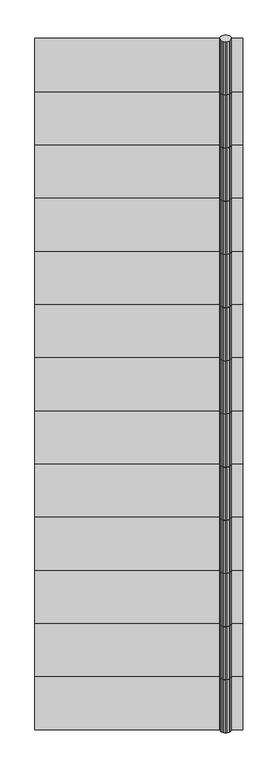
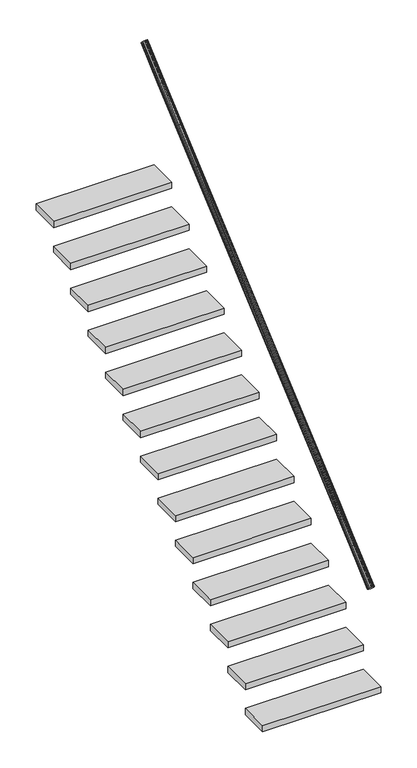
"""IFC4 building model written with IfcOpenShell, lengths in millimetres: stair geometry, 0_3d_modell."""

from ifc_helpers import new_model, si_unit, frame, origin, origin_with_axes, place, context, project, spatial, polyline, outline, extrude, source, transform, mapped, element, save


def stair_8bb973e3(model_context):
    return source(origin(), model_context, "Body", "SweptSolid", [
        extrude(outline(polyline([(1.2235871, -7.0656631), (0.0, 0.0), (1.2235871, 7.065663), (4.7745751, 13.4396897), (10.3053687, 18.498146), (17.2745751, 21.7458748), (25.0, 22.8649659), (32.7254249, 21.7458748), (39.6946313, 18.498146), (45.2254249, 13.4396897), (48.7764129, 7.065663), (50.0, 0.0), (48.7764129, -7.0656631), (45.2254249, -13.4396898), (39.6946313, -18.498146), (32.7254249, -21.7458748), (25.0, -22.8649659), (17.2745751, -21.7458748), (10.3053687, -18.498146), (4.7745751, -13.4396898), (1.2235871, -7.0656631)])), frame((850.0, 2774.9421971, 3252.4163795), z_axis=(0.0, 0.7569287102857436, 0.6534974579485071), x_axis=(-1.0, 0.0, 0.0)), (0.0, 0.0, 1.0), 303.8595272),
        extrude(outline(polyline([(0.0, 1164.9421971), (0.0, 1394.9421971), (900.0, 1394.9421971), (900.0, 1164.9421971), (0.0, 1164.9421971)])), frame((0.0, 0.0, 992.8571429), z_axis=(0.0, 0.0, 1.0), x_axis=(1.0, 0.0, 0.0)), (0.0, 0.0, 1.0), 50.0),
        extrude(outline(polyline([(0.0, 2544.9421971), (0.0, 2774.9421971), (900.0, 2774.9421971), (900.0, 2544.9421971), (0.0, 2544.9421971)])), frame((0.0, 0.0, 2184.2857143), z_axis=(0.0, 0.0, 1.0), x_axis=(1.0, 0.0, 0.0)), (0.0, 0.0, 1.0), 50.0),
        extrude(outline(polyline([(1.2235871, -7.0656631), (0.0, 0.0), (1.2235871, 7.065663), (4.7745751, 13.4396897), (10.3053687, 18.498146), (17.2745751, 21.7458748), (25.0, 22.8649659), (32.7254249, 21.7458748), (39.6946313, 18.498146), (45.2254249, 13.4396897), (48.7764129, 7.065663), (50.0, 0.0), (48.7764129, -7.0656631), (45.2254249, -13.4396897), (39.6946313, -18.498146), (32.7254249, -21.7458748), (25.0, -22.8649659), (17.2745751, -21.7458748), (10.3053687, -18.498146), (4.7745751, -13.4396897), (1.2235871, -7.0656631)])), frame((850.0, 1624.9421971, 2259.5592366), z_axis=(0.0, 0.7569287102856869, 0.653497457948573), x_axis=(-1.0, 0.0, 0.0)), (0.0, 0.0, 1.0), 303.8595272),
        extrude(outline(polyline([(1.2235871, -7.0656631), (0.0, 0.0), (1.2235871, 7.065663), (4.7745751, 13.4396898), (10.3053687, 18.498146), (17.2745751, 21.7458748), (25.0, 22.8649659), (32.7254249, 21.7458748), (39.6946313, 18.498146), (45.2254249, 13.4396898), (48.7764129, 7.065663), (50.0, 0.0), (48.7764129, -7.0656631), (45.2254249, -13.4396897), (39.6946313, -18.498146), (32.7254249, -21.7458748), (25.0, -22.8649659), (17.2745751, -21.7458748), (10.3053687, -18.498146), (4.7745751, -13.4396897), (1.2235871, -7.0656631)])), frame((850.0, 704.9421971, 1465.2735223), z_axis=(0.0, 0.7569287102857089, 0.6534974579485475), x_axis=(-1.0, 0.0, 0.0)), (0.0, 0.0, 1.0), 303.8595272),
        extrude(outline(polyline([(0.0, 244.9421971), (0.0, 474.9421971), (900.0, 474.9421971), (900.0, 244.9421971), (0.0, 244.9421971)])), frame((0.0, 0.0, 198.5714286), z_axis=(0.0, 0.0, 1.0), x_axis=(1.0, 0.0, 0.0)), (0.0, 0.0, 1.0), 50.0),
        extrude(outline(polyline([(0.0, 1624.9421971), (0.0, 1854.9421971), (900.0, 1854.9421971), (900.0, 1624.9421971), (0.0, 1624.9421971)])), frame((0.0, 0.0, 1390.0), z_axis=(0.0, 0.0, 1.0), x_axis=(1.0, 0.0, 0.0)), (0.0, 0.0, 1.0), 50.0),
        extrude(outline(polyline([(1.2235871, -7.0656631), (0.0, 0.0), (1.2235871, 7.065663), (4.7745751, 13.4396897), (10.3053687, 18.498146), (17.2745751, 21.7458748), (25.0, 22.8649659), (32.7254249, 21.7458748), (39.6946313, 18.498146), (45.2254249, 13.4396897), (48.7764129, 7.065663), (50.0, 0.0), (48.7764129, -7.0656631), (45.2254249, -13.4396898), (39.6946313, -18.498146), (32.7254249, -21.7458748), (25.0, -22.8649659), (17.2745751, -21.7458748), (10.3053687, -18.498146), (4.7745751, -13.4396898), (1.2235871, -7.0656631)])), frame((850.0, 934.9421971, 1663.8449509), z_axis=(0.0, 0.7569287102857098, 0.6534974579485463), x_axis=(-1.0, 0.0, 0.0)), (0.0, 0.0, 1.0), 303.8595272),
        extrude(outline(polyline([(1.2235871, -7.0656631), (0.0, 0.0), (1.2235871, 7.0656631), (4.7745751, 13.4396898), (10.3053687, 18.4981461), (17.2745751, 21.7458748), (25.0, 22.8649659), (32.7254249, 21.7458748), (39.6946313, 18.4981461), (45.2254249, 13.4396898), (48.7764129, 7.0656631), (50.0, 0.0), (48.7764129, -7.0656631), (45.2254249, -13.4396897), (39.6946313, -18.498146), (32.7254249, -21.7458748), (25.0, -22.8649659), (17.2745751, -21.7458748), (10.3053687, -18.498146), (4.7745751, -13.4396897), (1.2235871, -7.0656631)])), frame((850.0, 2084.9421971, 2656.7020937), z_axis=(0.0, 0.7569287102856951, 0.6534974579485633), x_axis=(-1.0, 0.0, 0.0)), (0.0, 0.0, 1.0), 303.8595272),
        extrude(outline(polyline([(0.0, 474.9421971), (0.0, 704.9421971), (900.0, 704.9421971), (900.0, 474.9421971), (0.0, 474.9421971)])), frame((0.0, 0.0, 397.1428571), z_axis=(0.0, 0.0, 1.0), x_axis=(1.0, 0.0, 0.0)), (0.0, 0.0, 1.0), 50.0),
        extrude(outline(polyline([(0.0, 2774.9421971), (0.0, 3004.9421971), (900.0, 3004.9421971), (900.0, 2774.9421971), (0.0, 2774.9421971)])), frame((0.0, 0.0, 2382.8571429), z_axis=(0.0, 0.0, 1.0), x_axis=(1.0, 0.0, 0.0)), (0.0, 0.0, 1.0), 50.0),
        extrude(outline(polyline([(0.0, 704.9421971), (0.0, 934.9421971), (900.0, 934.9421971), (900.0, 704.9421971), (0.0, 704.9421971)])), frame((0.0, 0.0, 595.7142857), z_axis=(0.0, 0.0, 1.0), x_axis=(1.0, 0.0, 0.0)), (0.0, 0.0, 1.0), 50.0),
        extrude(outline(polyline([(0.0, 934.9421971), (0.0, 1164.9421971), (900.0, 1164.9421971), (900.0, 934.9421971), (0.0, 934.9421971)])), frame((0.0, 0.0, 794.2857143), z_axis=(0.0, 0.0, 1.0), x_axis=(1.0, 0.0, 0.0)), (0.0, 0.0, 1.0), 50.0),
        extrude(outline(polyline([(1.2235871, -7.0656631), (0.0, 0.0), (1.2235871, 7.065663), (4.7745751, 13.4396897), (10.3053687, 18.498146), (17.2745751, 21.7458748), (25.0, 22.8649659), (32.7254249, 21.7458748), (39.6946313, 18.498146), (45.2254249, 13.4396897), (48.7764129, 7.065663), (50.0, 0.0), (48.7764129, -7.0656631), (45.2254249, -13.4396897), (39.6946313, -18.498146), (32.7254249, -21.7458748), (25.0, -22.8649659), (17.2745751, -21.7458748), (10.3053687, -18.498146), (4.7745751, -13.4396897), (1.2235871, -7.0656631)])), frame((850.0, 14.9421971, 869.5592366), z_axis=(0.0, 0.7569287102857067, 0.6534974579485499), x_axis=(-1.0, 0.0, 0.0)), (0.0, 0.0, 1.0), 303.8595272),
        extrude(outline(polyline([(1.2235871, -7.0656631), (0.0, 0.0), (1.2235871, 7.065663), (4.7745751, 13.4396897), (10.3053687, 18.498146), (17.2745751, 21.7458748), (25.0, 22.8649659), (32.7254249, 21.7458748), (39.6946313, 18.498146), (45.2254249, 13.4396897), (48.7764129, 7.065663), (50.0, 0.0), (48.7764129, -7.0656631), (45.2254249, -13.4396898), (39.6946313, -18.498146), (32.7254249, -21.7458748), (25.0, -22.8649659), (17.2745751, -21.7458748), (10.3053687, -18.498146), (4.7745751, -13.4396898), (1.2235871, -7.0656631)])), frame((850.0, 1854.9421971, 2458.1306652), z_axis=(0.0, 0.7569287102857034, 0.6534974579485536), x_axis=(-1.0, 0.0, 0.0)), (0.0, 0.0, 1.0), 303.8595272),
        extrude(outline(polyline([(0.0, 2314.9421971), (0.0, 2544.9421971), (900.0, 2544.9421971), (900.0, 2314.9421971), (0.0, 2314.9421971)])), frame((0.0, 0.0, 1985.7142857), z_axis=(0.0, 0.0, 1.0), x_axis=(1.0, 0.0, 0.0)), (0.0, 0.0, 1.0), 50.0),
        extrude(outline(polyline([(1.2235871, -7.0656631), (0.0, 0.0), (1.2235871, 7.0656631), (4.7745751, 13.4396898), (10.3053687, 18.498146), (17.2745751, 21.7458748), (25.0, 22.8649659), (32.7254249, 21.7458748), (39.6946313, 18.498146), (45.2254249, 13.4396898), (48.7764129, 7.0656631), (50.0, 0.0), (48.7764129, -7.0656631), (45.2254249, -13.4396897), (39.6946313, -18.498146), (32.7254249, -21.7458748), (25.0, -22.8649659), (17.2745751, -21.7458748), (10.3053687, -18.498146), (4.7745751, -13.4396897), (1.2235871, -7.0656631)])), frame((850.0, 1394.9421971, 2060.987808), z_axis=(0.0, 0.7569287102857012, 0.6534974579485563), x_axis=(-1.0, 0.0, 0.0)), (0.0, 0.0, 1.0), 303.8595272),
        extrude(outline(polyline([(1.2235871, -7.0656631), (0.0, 0.0), (1.2235871, 7.065663), (4.7745751, 13.4396898), (10.3053687, 18.498146), (17.2745751, 21.7458748), (25.0, 22.8649659), (32.7254249, 21.7458748), (39.6946313, 18.498146), (45.2254249, 13.4396898), (48.7764129, 7.065663), (50.0, 0.0), (48.7764129, -7.0656631), (45.2254249, -13.4396897), (39.6946313, -18.498146), (32.7254249, -21.7458748), (25.0, -22.8649659), (17.2745751, -21.7458748), (10.3053687, -18.498146), (4.7745751, -13.4396897), (1.2235871, -7.0656631)])), frame((850.0, 2314.9421971, 2855.2735223), z_axis=(0.0, 0.7569287102856991, 0.6534974579485587), x_axis=(-1.0, 0.0, 0.0)), (0.0, 0.0, 1.0), 303.8595272),
        extrude(outline(polyline([(1.2235871, -7.0656631), (0.0, 0.0), (1.2235871, 7.0656631), (4.7745751, 13.4396898), (10.3053687, 18.4981461), (17.2745751, 21.7458748), (25.0, 22.8649659), (32.7254249, 21.7458748), (39.6946313, 18.4981461), (45.2254249, 13.4396898), (48.7764129, 7.0656631), (50.0, 0.0), (48.7764129, -7.0656631), (45.2254249, -13.4396897), (39.6946313, -18.498146), (32.7254249, -21.7458748), (25.0, -22.8649659), (17.2745751, -21.7458748), (10.3053687, -18.498146), (4.7745751, -13.4396897), (1.2235871, -7.0656631)])), frame((850.0, 474.9421971, 1266.7020937), z_axis=(0.0, 0.7569287102857089, 0.6534974579485475), x_axis=(-1.0, 0.0, 0.0)), (0.0, 0.0, 1.0), 303.8595272),
        extrude(outline(polyline([(0.0, 2084.9421971), (0.0, 2314.9421971), (900.0, 2314.9421971), (900.0, 2084.9421971), (0.0, 2084.9421971)])), frame((0.0, 0.0, 1787.1428571), z_axis=(0.0, 0.0, 1.0), x_axis=(1.0, 0.0, 0.0)), (0.0, 0.0, 1.0), 50.0),
        extrude(outline(polyline([(1.2235871, -7.0656631), (0.0, 0.0), (1.2235871, 7.065663), (4.7745751, 13.4396897), (10.3053687, 18.498146), (17.2745751, 21.7458748), (25.0, 22.8649659), (32.7254249, 21.7458748), (39.6946313, 18.498146), (45.2254249, 13.4396897), (48.7764129, 7.065663), (50.0, 0.0), (48.7764129, -7.0656631), (45.2254249, -13.4396898), (39.6946313, -18.498146), (32.7254249, -21.7458748), (25.0, -22.8649659), (17.2745751, -21.7458748), (10.3053687, -18.498146), (4.7745751, -13.4396898), (1.2235871, -7.0656631)])), frame((850.0, 1164.9421971, 1862.4163795), z_axis=(0.0, 0.7569287102857021, 0.6534974579485554), x_axis=(-1.0, 0.0, 0.0)), (0.0, 0.0, 1.0), 303.8595272),
        extrude(outline(polyline([(0.0, 1854.9421971), (0.0, 2084.9421971), (900.0, 2084.9421971), (900.0, 1854.9421971), (0.0, 1854.9421971)])), frame((0.0, 0.0, 1588.5714286), z_axis=(0.0, 0.0, 1.0), x_axis=(1.0, 0.0, 0.0)), (0.0, 0.0, 1.0), 50.0),
        extrude(outline(polyline([(1.2235871, -7.0656631), (0.0, 0.0), (1.2235871, 7.065663), (4.7745751, 13.4396897), (10.3053687, 18.498146), (17.2745751, 21.7458748), (25.0, 22.8649659), (32.7254249, 21.7458748), (39.6946313, 18.498146), (45.2254249, 13.4396897), (48.7764129, 7.065663), (50.0, 0.0), (48.7764129, -7.0656631), (45.2254249, -13.4396898), (39.6946313, -18.498146), (32.7254249, -21.7458748), (25.0, -22.8649659), (17.2745751, -21.7458748), (10.3053687, -18.498146), (4.7745751, -13.4396898), (1.2235871, -7.0656631)])), frame((850.0, 2544.9421971, 3053.8449509), z_axis=(0.0, 0.7569287102857051, 0.6534974579485517), x_axis=(-1.0, 0.0, 0.0)), (0.0, 0.0, 1.0), 303.8595272),
        extrude(outline(polyline([(0.0, 1394.9421971), (0.0, 1624.9421971), (900.0, 1624.9421971), (900.0, 1394.9421971), (0.0, 1394.9421971)])), frame((0.0, 0.0, 1191.4285714), z_axis=(0.0, 0.0, 1.0), x_axis=(1.0, 0.0, 0.0)), (0.0, 0.0, 1.0), 50.0),
        extrude(outline(polyline([(1.2235871, -7.0656631), (0.0, 0.0), (1.2235871, 7.065663), (4.7745751, 13.4396897), (10.3053687, 18.498146), (17.2745751, 21.7458748), (25.0, 22.8649659), (32.7254249, 21.7458748), (39.6946313, 18.498146), (45.2254249, 13.4396897), (48.7764129, 7.065663), (50.0, 0.0), (48.7764129, -7.0656631), (45.2254249, -13.4396898), (39.6946313, -18.498146), (32.7254249, -21.7458748), (25.0, -22.8649659), (17.2745751, -21.7458748), (10.3053687, -18.498146), (4.7745751, -13.4396898), (1.2235871, -7.0656631)])), frame((850.0, 244.9421971, 1068.1306652), z_axis=(0.0, 0.7569287102856895, 0.6534974579485698), x_axis=(-1.0, 0.0, 0.0)), (0.0, 0.0, 1.0), 303.8595272),
        extrude(outline(polyline([(0.0, 14.9421971), (0.0, 244.9421971), (900.0, 244.9421971), (900.0, 14.9421971), (0.0, 14.9421971)])), origin_with_axes(), (0.0, 0.0, 1.0), 50.0),
    ])


if __name__ == "__main__":
    model = new_model("IFC4")
    model_context = context("Model", 3, world=origin())
    ifc_project = project(units=[si_unit("LENGTHUNIT", "METRE", prefix="MILLI")], contexts=[model_context])
    site = spatial("IfcSite", under=ifc_project)
    building = spatial("IfcBuilding", under=site)
    placement = place(None, origin())
    stair_shape = stair_8bb973e3(model_context)
    element("IfcStair", 1, ObjectType="0_3d_modell", at=placement, inside=building, context=model_context, shape_type="MappedRepresentation", body=[
        mapped(stair_shape, transform((0.0, 0.0, 0.0), x_axis=(1.0, 0.0, 0.0), y_axis=(0.0, 1.0, 0.0), z_axis=(0.0, 0.0, 1.0))),
    ])
    save(model, "model.ifc")

# Revit data of these elements
# Element 1 (IfcStair, "0_3d_modell")
#   Materials on its faces: "*1", "weiss"
# Materials
#   "*1": class "Unassigned", colour RGB 175 175 175, transparency 0
#   "weiss": class "Unassigned", colour RGB 255 255 255, transparency 0
